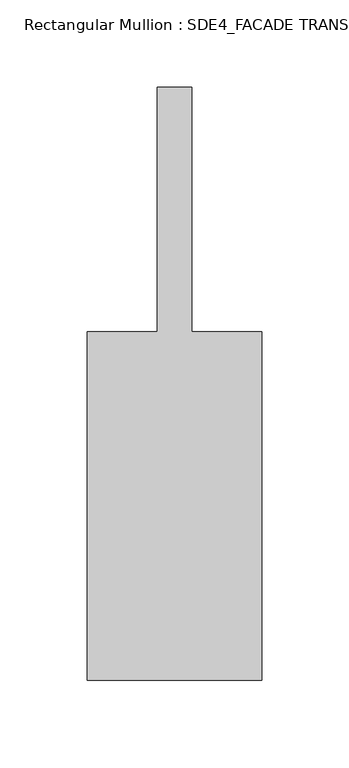
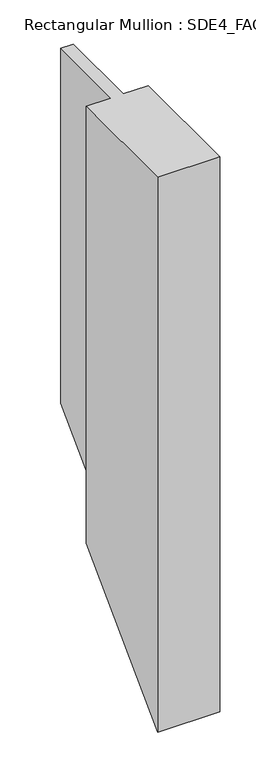
"""IFC4 building model written with IfcOpenShell, lengths in millimetres: member geometry, Rectangular Mullion : SDE4_FACADE TRANSOM TYPE 1."""

from ifc_helpers import new_model, si_unit, origin, place, context, project, spatial, faceted_brep, source, transform, mapped, element, save


def rectangular_mullion_sde4_facade_transom_type_1_ffd698e1(model_context):
    return source(origin(), model_context, "Body", "Brep", [
        faceted_brep([(50.0, -132.5, 0.0), (50.0, 67.5, 0.0), (10.0, 67.5, 0.0), (10.0, 207.5, 0.0), (-10.0, 207.5, 0.0), (-10.0, 67.5, 0.0), (-50.0, 67.5, 0.0), (-50.0, -132.5, 0.0), (50.0, -132.5, -944.6197543), (50.0, 67.5, -744.6197543), (10.0, 67.5, -744.6197543), (10.0, 207.5, -604.6197543), (-10.0, 207.5, -604.6197543), (-10.0, 67.5, -744.6197543), (-50.0, 67.5, -744.6197543), (-50.0, -132.5, -944.6197543)], [[[0, 1, 2, 3, 4, 5, 6, 7]], [[1, 0, 8, 9]], [[2, 1, 9, 10]], [[3, 2, 10, 11]], [[4, 3, 11, 12]], [[5, 4, 12, 13]], [[6, 5, 13, 14]], [[7, 6, 14, 15]], [[0, 7, 15, 8]], [[8, 15, 14, 13, 12, 11, 10, 9]]]),
    ])


if __name__ == "__main__":
    model = new_model("IFC4")
    model_context = context("Model", 3, world=origin())
    ifc_project = project(units=[si_unit("LENGTHUNIT", "METRE", prefix="MILLI")], contexts=[model_context])
    site = spatial("IfcSite", under=ifc_project)
    building = spatial("IfcBuilding", under=site)
    placement = place(None, origin())
    rectangular_mullion_sde4_facade_transom_type_1_shape = rectangular_mullion_sde4_facade_transom_type_1_ffd698e1(model_context)
    element("IfcMember", 1, ObjectType="Rectangular Mullion : SDE4_FACADE TRANSOM TYPE 1", at=placement, inside=building, context=model_context, shape_type="MappedRepresentation", body=[
        mapped(rectangular_mullion_sde4_facade_transom_type_1_shape, transform((0.0, 0.0, 0.0), x_axis=(1.0, 0.0, 0.0), y_axis=(0.0, 1.0, 0.0), z_axis=(0.0, 0.0, 1.0))),
    ])
    save(model, "model.ifc")

# Revit data of these elements
# Type "Rectangular Mullion : SDE4_FACADE TRANSOM TYPE 1"
#   built-in parameter 1007322 = 1.11549 (stored number, unit not read)
#   built-in parameter 1007321 = 0.164042 (stored number, unit not read)
#   built-in parameter 1007320 = 0.164042 (stored number, unit not read)
